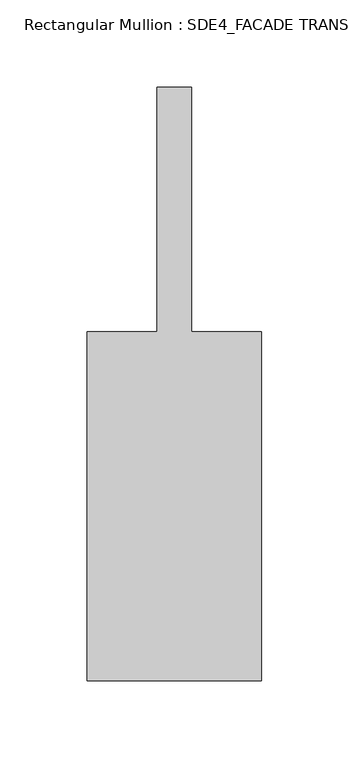
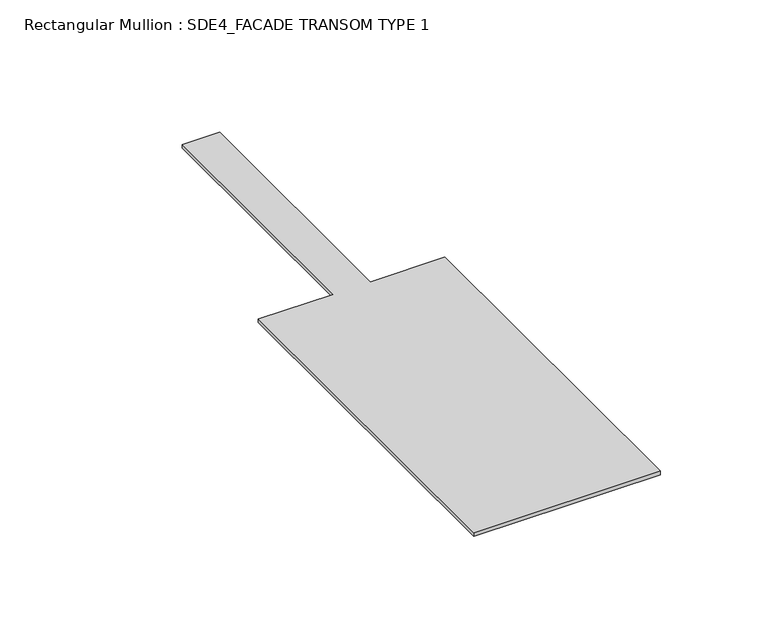
"""IFC4 building model written with IfcOpenShell, lengths in millimetres: member geometry, Rectangular Mullion : SDE4_FACADE TRANSOM TYPE 1."""

import ifcopenshell
import ifcopenshell.guid

model = None  # the IFC model being written
_history = None  # IfcOwnerHistory: only IFC2X3 demands one
_inside = {}  # id of a spatial element -> (the spatial element, [elements in it])
_under = {}  # id of a project, library or spatial element -> (it, [spatial elements below it])
_declared = {}  # id of a project -> (the project, [libraries it declares])
_typed = {}  # id of a type object -> (the type object, [elements of that type])
_made_of = {}  # id of a material, layer set ... -> (it, [elements and type objects made of it])


def new_model(schema):
    """Start an empty IFC model of exactly this schema.

    Asked for "IFC4X3", IfcOpenShell would pick the latest addendum, in which some entities
    have other attributes; the version numbers below select the first issue.
    IFC2X3 requires an IfcOwnerHistory on every rooted entity: one is made here for all.
    """
    global model, _history
    if schema == "IFC4X3":
        model = ifcopenshell.file(schema_version=(4, 3, 0, 0))
    else:
        model = ifcopenshell.file(schema=schema)
    _inside.clear()
    _under.clear()
    _declared.clear()
    _typed.clear()
    _made_of.clear()
    _history = None
    if model.schema == "IFC2X3":
        org = make("IfcOrganization", Name="unknown")
        user = make(
            "IfcPersonAndOrganization",
            ThePerson=make("IfcPerson", FamilyName="unknown"),
            TheOrganization=org,
        )
        app = make(
            "IfcApplication",
            ApplicationDeveloper=org,
            Version="unknown",
            ApplicationFullName="unknown",
            ApplicationIdentifier="unknown",
        )
        _history = make(
            "IfcOwnerHistory",
            OwningUser=user,
            OwningApplication=app,
            ChangeAction="ADDED",
            CreationDate=0,
        )
    return model


def make(cls, **values):
    """One entity of the class cls with the attributes given. An attribute that is None is left unset."""
    return model.create_entity(
        cls, **{name: value for name, value in values.items() if value is not None}
    )


def rooted(cls, **values):
    """An entity with a GlobalId (a new one), such as an element, a storey or a relation."""
    return make(cls, GlobalId=ifcopenshell.guid.new(), OwnerHistory=_history, **values)


def si_unit(unit_type, name, prefix=None):
    """IfcSIUnit, for example si_unit("LENGTHUNIT", "METRE", prefix="MILLI")."""
    return make("IfcSIUnit", UnitType=unit_type, Prefix=prefix, Name=name)


def assignment(units):
    """IfcUnitAssignment: the units of a project."""
    return None if units is None else make("IfcUnitAssignment", Units=units)


def point(xyz):
    """IfcCartesianPoint."""
    return None if xyz is None else make("IfcCartesianPoint", Coordinates=xyz)


def direction(xyz):
    """IfcDirection."""
    return None if xyz is None else make("IfcDirection", DirectionRatios=xyz)


def frame(location, z_axis=None, x_axis=None):
    """IfcAxis2Placement3D, a coordinate frame: its origin and axes. An axis left out is left unset."""
    return make(
        "IfcAxis2Placement3D",
        Location=point(location),
        Axis=direction(z_axis),
        RefDirection=direction(x_axis),
    )


def origin():
    """The frame at (0, 0, 0) with its axes left unset."""
    return frame((0.0, 0.0, 0.0))


def place(relative_to, where):
    """IfcLocalPlacement: puts the frame where relative to a parent placement (None: the world)."""
    return make(
        "IfcLocalPlacement", PlacementRelTo=relative_to, RelativePlacement=where
    )


def context(
    kind, dimensions, precision=None, world=None, true_north=None, identifier=None
):
    """IfcGeometricRepresentationContext, for example the 3D "Model" context."""
    return make(
        "IfcGeometricRepresentationContext",
        ContextIdentifier=identifier,
        ContextType=kind,
        CoordinateSpaceDimension=dimensions,
        Precision=precision,
        WorldCoordinateSystem=world,
        TrueNorth=true_north,
    )


def project(units=None, contexts=None):
    """IfcProject with its units and contexts."""
    return rooted(
        "IfcProject",
        Name="project",
        RepresentationContexts=contexts,
        UnitsInContext=assignment(units),
    )


def spatial(cls, under=None, at=None, **own):
    """A site, building, storey or space (cls), placed at a placement, below another one or the project."""
    s = rooted(cls, ObjectPlacement=at, **own)
    if under is not None:
        _under.setdefault(under.id(), (under, []))[1].append(s)
    return s


def polyline(points):
    """IfcPolyline through the points."""
    return make("IfcPolyline", Points=[point(p) for p in points])


def outline(outer, holes=None, kind="AREA"):
    """IfcArbitraryClosedProfileDef: a profile drawn as a closed curve; with holes, ...WithVoids."""
    if holes is None:
        return make("IfcArbitraryClosedProfileDef", ProfileType=kind, OuterCurve=outer)
    return make(
        "IfcArbitraryProfileDefWithVoids",
        ProfileType=kind,
        OuterCurve=outer,
        InnerCurves=holes,
    )


def extrude(swept, where, along, depth):
    """IfcExtrudedAreaSolid: the profile swept, set in the frame where, extruded along a direction by depth."""
    return make(
        "IfcExtrudedAreaSolid",
        SweptArea=swept,
        Position=where,
        ExtrudedDirection=direction(along),
        Depth=depth,
    )


def shape(context_of_items, identifier, shape_type, items):
    """IfcShapeRepresentation: the items that make up one representation, for example the "Body"."""
    return make(
        "IfcShapeRepresentation",
        ContextOfItems=context_of_items,
        RepresentationIdentifier=identifier,
        RepresentationType=shape_type,
        Items=items,
    )


def source(mapping_origin, context_of_items, identifier, shape_type, items):
    """IfcRepresentationMap: a shape defined once, which mapped items show again and again."""
    return make(
        "IfcRepresentationMap",
        MappingOrigin=mapping_origin,
        MappedRepresentation=shape(context_of_items, identifier, shape_type, items),
    )


def transform(
    local_origin,
    x_axis=None,
    y_axis=None,
    z_axis=None,
    scale=None,
    scale2=None,
    scale3=None,
    uniform=True,
):
    """IfcCartesianTransformationOperator3D, or its non-uniform kind. x_axis, y_axis, z_axis: its Axis1, 2, 3."""
    if uniform:
        return make(
            "IfcCartesianTransformationOperator3D",
            Axis1=direction(x_axis),
            Axis2=direction(y_axis),
            LocalOrigin=point(local_origin),
            Scale=scale,
            Axis3=direction(z_axis),
        )
    return make(
        "IfcCartesianTransformationOperator3DnonUniform",
        Axis1=direction(x_axis),
        Axis2=direction(y_axis),
        LocalOrigin=point(local_origin),
        Scale=scale,
        Axis3=direction(z_axis),
        Scale2=scale2,
        Scale3=scale3,
    )


def mapped(mapping_source, mapping_target):
    """IfcMappedItem: shows the shape of a source again, moved by a transform."""
    return make(
        "IfcMappedItem", MappingSource=mapping_source, MappingTarget=mapping_target
    )


def made_of(thing, what):
    """Note that an element or type object is made of a material, layer set ...; save() writes the relation."""
    if what is not None:
        _made_of.setdefault(what.id(), (what, []))[1].append(thing)
    return thing


def element(
    cls,
    number,
    at=None,
    inside=None,
    cuts=None,
    type_object=None,
    material=None,
    context=None,
    identifier="Body",
    shape_type=None,
    held_by="IfcProductDefinitionShape",
    body=None,
    shapes=None,
    **own,
):
    """One element of the class cls, such as IfcWall. Its Tag is "e" and its number.

    at: its placement. inside: the storey or other place that contains it. cuts: it is an
    opening in that element (IfcRelVoidsElement). A single representation is given by context,
    identifier, shape_type and body (its items); several are given by shapes. held_by: the class
    of the entity that holds the representations. save() writes the other relations.
    """
    e = rooted(cls, Tag="e%d" % number, ObjectPlacement=at, **own)
    if body is not None:
        shapes = [shape(context, identifier, shape_type, body)]
    if shapes is not None:
        e.Representation = make(held_by, Representations=shapes)
    if inside is not None:
        _inside.setdefault(inside.id(), (inside, []))[1].append(e)
    if cuts is not None:
        rooted(
            "IfcRelVoidsElement", RelatingBuildingElement=cuts, RelatedOpeningElement=e
        )
    if type_object is not None:
        _typed.setdefault(type_object.id(), (type_object, []))[1].append(e)
    return made_of(e, material)


def aggregate(whole, parts):
    """IfcRelAggregates: a whole, such as a stair, and the parts it consists of."""
    return rooted("IfcRelAggregates", RelatingObject=whole, RelatedObjects=parts)


def save(model, path):
    """Write the relations noted so far, then the file.

    IfcRelAggregates (storeys below a building ...), IfcRelContainedInSpatialStructure (elements
    in a storey), IfcRelDefinesByType, IfcRelAssociatesMaterial and IfcRelDeclares: one each for
    every whole, place, type object, material and project.
    """
    for whole, parts in _under.values():
        aggregate(whole, parts)
    for where, things in _inside.values():
        rooted(
            "IfcRelContainedInSpatialStructure",
            RelatedElements=things,
            RelatingStructure=where,
        )
    for kind, things in _typed.values():
        rooted("IfcRelDefinesByType", RelatedObjects=things, RelatingType=kind)
    for what, things in _made_of.values():
        rooted("IfcRelAssociatesMaterial", RelatedObjects=things, RelatingMaterial=what)
    for by, libraries in _declared.values():
        rooted("IfcRelDeclares", RelatingContext=by, RelatedDefinitions=libraries)
    model.write(path)


def rectangular_mullion_sde4_facade_transom_type_1_a5cd460e(model_context):
    return source(origin(), model_context, "Body", "SweptSolid", [
        extrude(outline(polyline([(50.0, -132.5), (-50.0, -132.5), (-50.0, 67.5), (-10.0, 67.5), (-10.0, 207.5), (10.0, 207.5), (10.0, 67.5), (50.0, 67.5), (50.0, -132.5)])), frame((0.0, 0.0, -2.0372978), z_axis=(0.0, 0.0, 1.0), x_axis=(1.0, 0.0, 0.0)), (0.0, 0.0, 1.0), 2.0372978),
    ])


if __name__ == "__main__":
    model = new_model("IFC4")
    model_context = context("Model", 3, world=origin())
    ifc_project = project(units=[si_unit("LENGTHUNIT", "METRE", prefix="MILLI")], contexts=[model_context])
    site = spatial("IfcSite", under=ifc_project)
    building = spatial("IfcBuilding", under=site)
    placement = place(None, origin())
    rectangular_mullion_sde4_facade_transom_type_1_shape = rectangular_mullion_sde4_facade_transom_type_1_a5cd460e(model_context)
    element("IfcMember", 1, ObjectType="Rectangular Mullion : SDE4_FACADE TRANSOM TYPE 1", at=placement, inside=building, context=model_context, shape_type="MappedRepresentation", body=[
        mapped(rectangular_mullion_sde4_facade_transom_type_1_shape, transform((0.0, 0.0, 0.0), x_axis=(1.0, 0.0, 0.0), y_axis=(0.0, 1.0, 0.0), z_axis=(0.0, 0.0, 1.0))),
    ])
    save(model, "model.ifc")

# Revit data of these elements
# Type "Rectangular Mullion : SDE4_FACADE TRANSOM TYPE 1"
#   built-in parameter 1007322 = 1.11549 (stored number, unit not read)
#   built-in parameter 1007321 = 0.164042 (stored number, unit not read)
#   built-in parameter 1007320 = 0.164042 (stored number, unit not read)
